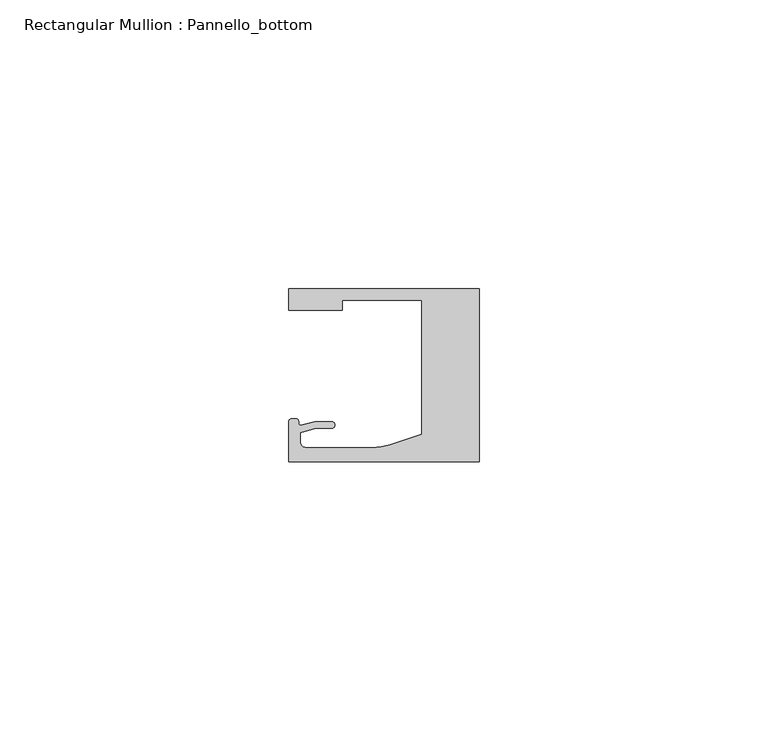
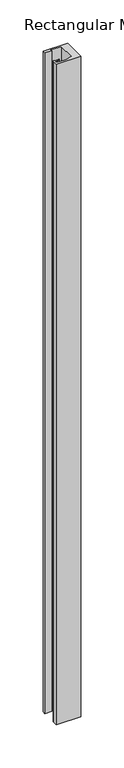
"""IFC4 building model written with IfcOpenShell, lengths in millimetres: member geometry, Rectangular Mullion : Pannello_bottom."""

from ifc_helpers import new_model, si_unit, frame, origin, place, context, project, spatial, polyline, circle_curve, source, transform, mapped, element, save
from ifc_brep_helpers import plane_surface, cylinder_surface, revolved_surface, extruded_surface, spline_curve, advanced_brep


def rectangular_mullion_pannello_bottom_8b902226(model_context):
    return source(origin(), model_context, "Body", "AdvancedBrep", [
        advanced_brep(
        [(-33.0, 15.0, 0.0), (-33.0, 11.3000004, 0.0), (-23.700041, 11.3000004, 0.0), (-23.700041, 13.0000004, 0.0), (-9.9999723, 13.0000004, 0.0), (-9.9999723, -10.2367227, 0.0), (-15.4591336, -12.0105099, 0.0), (-18.5493024, -12.4999438, 0.0), (-30.0000002, -12.4999419, 0.0), (-31.0, -11.4999419, 0.0), (-31.0, -9.9121746, 0.0), (-28.3419477, -9.1999523, 0.0), (-25.59998, -9.1999523, 0.0), (-25.59998, -7.9999523, 0.0), (-28.4999305, -7.9999523, 0.0), (-30.9223017, -8.6490241, 0.0), (-33.0000135, -8.0000472, 0.0), (-33.0000135, -15.0, 0.0), (0.0, -15.0, 0.0), (0.0, 15.0, 0.0), (-33.0, 15.0, -933.9999729), (0.0, 15.0, -933.9999729), (0.0, -15.0, -933.9999729), (-33.0000135, -15.0, -933.9999729), (-33.0000135, -8.0000472, -933.9999729), (-30.9223017, -8.6490241, -933.9999729), (-28.4999305, -7.9999523, -933.9999729), (-25.59998, -7.9999523, -933.9999729), (-25.59998, -9.1999523, -933.9999729), (-28.3419477, -9.1999523, -933.9999729), (-31.0, -9.9121746, -933.9999729), (-31.0, -11.4999419, -933.9999729), (-30.0000002, -12.4999419, -933.9999729), (-18.5493024, -12.4999438, -933.9999729), (-15.4591336, -12.0105099, -933.9999729), (-9.9999723, -10.2367227, -933.9999729), (-9.9999723, 13.0000004, -933.9999729), (-23.700041, 13.0000004, -933.9999729), (-23.700041, 11.3000004, -933.9999729), (-33.0, 11.3000004, -933.9999729)],
        [
            (0, 1),
            (1, 2),
            (2, 3),
            (3, 4),
            (4, 5),
            (5, 6),
            (6, 7, circle_curve(frame((-18.5493007, -2.4999438, 0.0), z_axis=(0.0, 0.0, -1.0), x_axis=(0.0, -1.0, 0.0)), 10.0)),
            (7, 8),
            (8, 9, circle_curve(frame((-30.0, -11.4999419, 0.0), z_axis=(0.0, 0.0, -1.0), x_axis=(0.0, -1.0, 0.0)), 1.0)),
            (9, 10),
            (10, 11),
            (11, 12),
            (12, 13, circle_curve(frame((-25.59998, -8.5999523, 0.0), z_axis=(0.0, 0.0, 1.0), x_axis=(0.0, -1.0, 0.0)), 0.6)),
            (13, 14),
            (14, 15),
            (15, 16, spline_curve(3, [(-30.9223017, -8.6490241, 0.0), (-31.312054066, -8.717747958, 0.0), (-31.298563602, -8.366228555, 0.0), (-31.305645054, -7.690065204, 0.0), (-31.357433266, -7.563996614, 0.0), (-32.262327879, -7.456527435, 0.0), (-33.0000135, -7.457047519, 0.0), (-33.0000135, -8.0000472, 0.0)], [4, 2, 2, 4], [0.0, 0.001840817752199412, 0.004996616814974408, 0.007702013405570312])),
            (16, 17),
            (17, 18),
            (18, 19),
            (19, 0),
            (20, 21),
            (21, 22),
            (22, 23),
            (23, 24),
            (24, 25, spline_curve(3, [(-33.0000135, -8.0000472, -933.9999729), (-33.0000135, -7.457047519, -933.9999729), (-32.262327879, -7.456527435, -933.9999729), (-31.357433266, -7.563996614, -933.9999729), (-31.305645054, -7.690065204, -933.9999729), (-31.298563602, -8.366228555, -933.9999729), (-31.312054066, -8.717747958, -933.9999729), (-30.9223017, -8.6490241, -933.9999729)], [4, 2, 2, 4], [0.0, 0.0027053965905959043, 0.0058611956533709, 0.007702013405570312])),
            (25, 26),
            (26, 27),
            (27, 28, circle_curve(frame((-25.59998, -8.5999523, -933.9999729), z_axis=(0.0, 0.0, -1.0), x_axis=(0.0, -1.0, 0.0)), 0.6)),
            (28, 29),
            (29, 30),
            (30, 31),
            (31, 32, circle_curve(frame((-30.0, -11.4999419, -933.9999729), z_axis=(0.0, 0.0, 1.0), x_axis=(0.0, -1.0, 0.0)), 1.0)),
            (32, 33),
            (33, 34, circle_curve(frame((-18.5493007, -2.4999438, -933.9999729), z_axis=(0.0, 0.0, 1.0), x_axis=(0.0, -1.0, 0.0)), 10.0)),
            (34, 35),
            (35, 36),
            (36, 37),
            (37, 38),
            (38, 39),
            (39, 20),
            (0, 20),
            (39, 1),
            (38, 2),
            (37, 3),
            (36, 4),
            (35, 5),
            (34, 6),
            (33, 7),
            (32, 8),
            (31, 9),
            (30, 10),
            (29, 11),
            (28, 12),
            (27, 13),
            (26, 14),
            (25, 15),
            (24, 16),
            (23, 17),
            (22, 18),
            (21, 19),
        ],
        [
            plane_surface(frame((0.0, -36.2491502, 0.0), z_axis=(0.0, 0.0, 1.0), x_axis=(-1.0, 0.0, 0.0))),
            plane_surface(frame((0.0, -36.2491502, -933.9999729), z_axis=(0.0, 0.0, -1.0), x_axis=(-1.0, 0.0, 0.0))),
            plane_surface(frame((-33.0, 15.0, 0.0), z_axis=(-1.0, 0.0, 0.0), x_axis=(0.0, 0.0, -1.0))),
            plane_surface(frame((-33.0, 11.3000004, 0.0), z_axis=(0.0, -1.0, 0.0), x_axis=(0.0, 0.0, -1.0))),
            plane_surface(frame((-23.700041, 11.3000004, 0.0), z_axis=(1.0, 0.0, 0.0), x_axis=(0.0, 0.0, -1.0))),
            plane_surface(frame((-23.700041, 13.0000004, 0.0), z_axis=(0.0, -1.0, 0.0), x_axis=(0.0, 0.0, -1.0))),
            plane_surface(frame((-9.9999723, 13.0000004, 0.0), z_axis=(-1.0, 0.0, 0.0), x_axis=(0.0, 0.0, -1.0))),
            plane_surface(frame((-9.9999723, -10.2367227, 0.0), z_axis=(-0.30901670911956314, 0.9510566089801992, 0.0), x_axis=(0.0, 0.0, -1.0))),
            revolved_surface(polyline([(-18.5493007, -12.4999438, -933.9999729), (-18.5493007, -12.4999438, 0.0)]), (-18.5493007, -2.4999438, 0.0), (0.0, 0.0, -1.0)),
            plane_surface(frame((-18.5493024, -12.4999438, 0.0), z_axis=(1.6923026533778639e-07, 0.9999999999999858, 0.0), x_axis=(0.0, 0.0, -1.0))),
            revolved_surface(polyline([(-30.0, -12.4999419, -933.9999729), (-30.0, -12.4999419, 0.0)]), (-30.0, -11.4999419, 0.0), (0.0, 0.0, -1.0)),
            plane_surface(frame((-31.0, -11.4999419, 0.0), z_axis=(1.0, 0.0, 0.0), x_axis=(0.0, 0.0, -1.0))),
            plane_surface(frame((-31.0, -9.9121746, 0.0), z_axis=(0.25881883204288636, -0.9659258833782002, 0.0), x_axis=(0.0, 0.0, -1.0))),
            plane_surface(frame((-28.3419477, -9.1999523, 0.0), z_axis=(0.0, -1.0, 0.0), x_axis=(0.0, 0.0, -1.0))),
            cylinder_surface(frame((-25.59998, -8.5999523, 0.0), z_axis=(0.0, 0.0, 1.0), x_axis=(0.0, -1.0, 0.0)), 0.6),
            plane_surface(frame((-25.59998, -7.9999523, 0.0), z_axis=(0.0, 1.0, 0.0), x_axis=(0.0, 0.0, -1.0))),
            plane_surface(frame((-28.4999305, -7.9999523, 0.0), z_axis=(-0.25881883200192934, 0.9659258833891746, 0.0), x_axis=(0.0, 0.0, -1.0))),
            extruded_surface(spline_curve(3, [(-30.9223017, -8.6490241, -933.9999729), (-31.312054066, -8.717747958, -933.9999729), (-31.298563602, -8.366228555, -933.9999729), (-31.305645054, -7.690065204, -933.9999729), (-31.357433266, -7.563996614, -933.9999729), (-32.262327879, -7.456527435, -933.9999729), (-33.0000135, -7.457047519, -933.9999729), (-33.0000135, -8.0000472, -933.9999729)], [4, 2, 2, 4], [0.0, 0.001840817752199412, 0.004996616814974408, 0.007702013405570312]), (0.0, 0.0, 933.9999729), 933.9999729),
            plane_surface(frame((-33.0000135, -8.0000472, 0.0), z_axis=(-1.0, 0.0, 0.0), x_axis=(0.0, 0.0, -1.0))),
            plane_surface(frame((-33.0000135, -15.0, 0.0), z_axis=(0.0, -1.0, 0.0), x_axis=(0.0, 0.0, -1.0))),
            plane_surface(frame((0.0, -15.0, 0.0), z_axis=(1.0, 0.0, 0.0), x_axis=(0.0, 0.0, -1.0))),
            plane_surface(frame((0.0, 15.0, 0.0), z_axis=(0.0, 1.0, 0.0), x_axis=(0.0, 0.0, -1.0))),
        ],
        [
            (0, [[1, 2, 3, 4, 5, 6, 7, 8, 9, 10, 11, 12, 13, 14, 15, 16, 17, 18, 19, 20]]),
            (1, [[21, 22, 23, 24, 25, 26, 27, 28, 29, 30, 31, 32, 33, 34, 35, 36, 37, 38, 39, 40]]),
            (2, [[-1, 41, -40, 42]]),
            (3, [[-2, -42, -39, 43]]),
            (4, [[-3, -43, -38, 44]]),
            (5, [[-4, -44, -37, 45]]),
            (6, [[-5, -45, -36, 46]]),
            (7, [[-6, -46, -35, 47]]),
            (8, [[-7, -47, -34, 48]]),
            (9, [[-8, -48, -33, 49]]),
            (10, [[-9, -49, -32, 50]]),
            (11, [[-10, -50, -31, 51]]),
            (12, [[-11, -51, -30, 52]]),
            (13, [[-12, -52, -29, 53]]),
            (14, [[-13, -53, -28, 54]]),
            (15, [[-14, -54, -27, 55]]),
            (16, [[-15, -55, -26, 56]]),
            (17, [[-16, -56, -25, 57]]),
            (18, [[-17, -57, -24, 58]]),
            (19, [[-18, -58, -23, 59]]),
            (20, [[-19, -59, -22, 60]]),
            (21, [[-20, -60, -21, -41]]),
        ],
    ),
    ])


if __name__ == "__main__":
    model = new_model("IFC4")
    model_context = context("Model", 3, world=origin())
    ifc_project = project(units=[si_unit("LENGTHUNIT", "METRE", prefix="MILLI")], contexts=[model_context])
    site = spatial("IfcSite", under=ifc_project)
    building = spatial("IfcBuilding", under=site)
    placement = place(None, origin())
    rectangular_mullion_pannello_bottom_shape = rectangular_mullion_pannello_bottom_8b902226(model_context)
    element("IfcMember", 1, ObjectType="Rectangular Mullion : Pannello_bottom", at=placement, inside=building, context=model_context, shape_type="MappedRepresentation", body=[
        mapped(rectangular_mullion_pannello_bottom_shape, transform((0.0, 0.0, 0.0), x_axis=(1.0, 0.0, 0.0), y_axis=(0.0, 1.0, 0.0), z_axis=(0.0, 0.0, 1.0))),
    ])
    save(model, "model.ifc")

# Revit data of these elements
# Type "Rectangular Mullion : Pannello_bottom"
#   built-in parameter 1007322 = 0.0984252 (stored number, unit not read)
#   built-in parameter 1007321 = 0.0328083 (stored number, unit not read)
#   built-in parameter 1007320 = 0 (stored number, unit not read)
